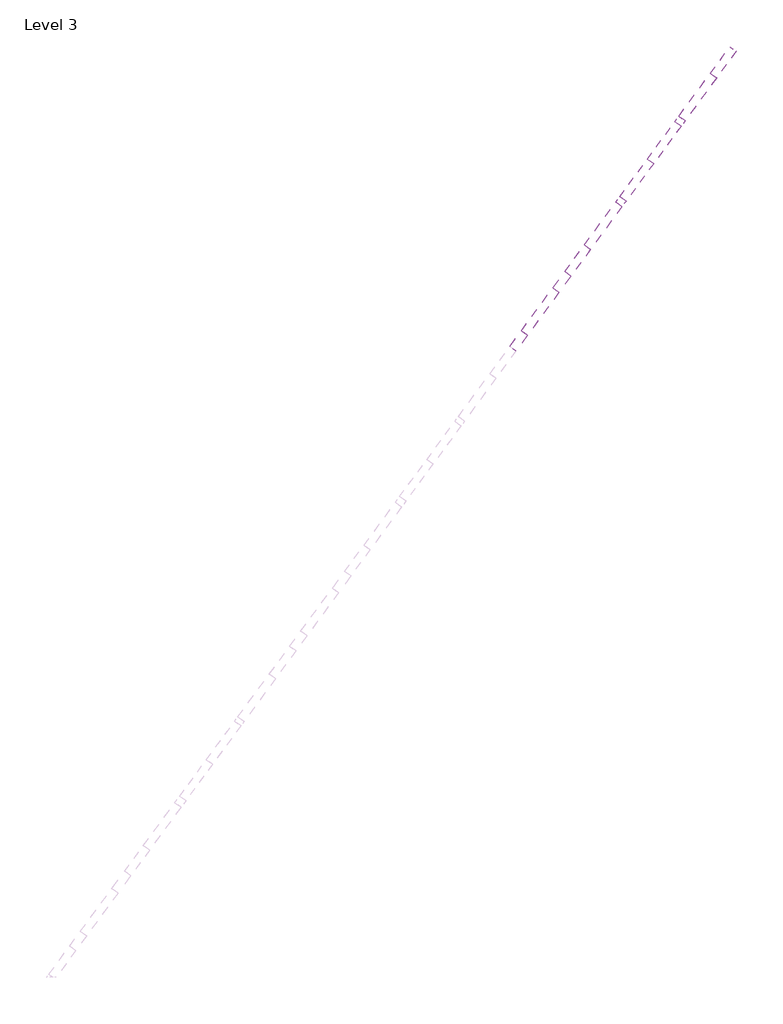
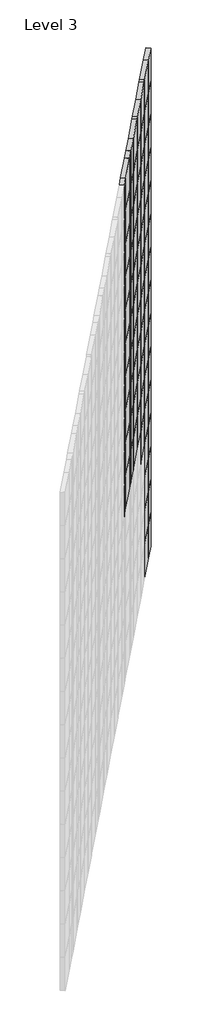
# One storey, part 9 of 9: 122 plates.
"""IFC4 building model written with IfcOpenShell, lengths in millimetres."""

import ifcopenshell
import ifcopenshell.guid

model = None  # the IFC model being written
_history = None  # IfcOwnerHistory: only IFC2X3 demands one
_inside = {}  # id of a spatial element -> (the spatial element, [elements in it])
_under = {}  # id of a project, library or spatial element -> (it, [spatial elements below it])
_declared = {}  # id of a project -> (the project, [libraries it declares])
_typed = {}  # id of a type object -> (the type object, [elements of that type])
_made_of = {}  # id of a material, layer set ... -> (it, [elements and type objects made of it])


def new_model(schema):
    """Start an empty IFC model of exactly this schema.

    Asked for "IFC4X3", IfcOpenShell would pick the latest addendum, in which some entities
    have other attributes; the version numbers below select the first issue.
    IFC2X3 requires an IfcOwnerHistory on every rooted entity: one is made here for all.
    """
    global model, _history
    if schema == "IFC4X3":
        model = ifcopenshell.file(schema_version=(4, 3, 0, 0))
    else:
        model = ifcopenshell.file(schema=schema)
    _inside.clear()
    _under.clear()
    _declared.clear()
    _typed.clear()
    _made_of.clear()
    _history = None
    if model.schema == "IFC2X3":
        org = make("IfcOrganization", Name="unknown")
        user = make(
            "IfcPersonAndOrganization",
            ThePerson=make("IfcPerson", FamilyName="unknown"),
            TheOrganization=org,
        )
        app = make(
            "IfcApplication",
            ApplicationDeveloper=org,
            Version="unknown",
            ApplicationFullName="unknown",
            ApplicationIdentifier="unknown",
        )
        _history = make(
            "IfcOwnerHistory",
            OwningUser=user,
            OwningApplication=app,
            ChangeAction="ADDED",
            CreationDate=0,
        )
    return model


def make(cls, **values):
    """One entity of the class cls with the attributes given. An attribute that is None is left unset."""
    return model.create_entity(
        cls, **{name: value for name, value in values.items() if value is not None}
    )


def rooted(cls, **values):
    """An entity with a GlobalId (a new one), such as an element, a storey or a relation."""
    return make(cls, GlobalId=ifcopenshell.guid.new(), OwnerHistory=_history, **values)


def si_unit(unit_type, name, prefix=None):
    """IfcSIUnit, for example si_unit("LENGTHUNIT", "METRE", prefix="MILLI")."""
    return make("IfcSIUnit", UnitType=unit_type, Prefix=prefix, Name=name)


def assignment(units):
    """IfcUnitAssignment: the units of a project."""
    return None if units is None else make("IfcUnitAssignment", Units=units)


def point(xyz):
    """IfcCartesianPoint."""
    return None if xyz is None else make("IfcCartesianPoint", Coordinates=xyz)


def direction(xyz):
    """IfcDirection."""
    return None if xyz is None else make("IfcDirection", DirectionRatios=xyz)


def frame(location, z_axis=None, x_axis=None):
    """IfcAxis2Placement3D, a coordinate frame: its origin and axes. An axis left out is left unset."""
    return make(
        "IfcAxis2Placement3D",
        Location=point(location),
        Axis=direction(z_axis),
        RefDirection=direction(x_axis),
    )


def origin():
    """The frame at (0, 0, 0) with its axes left unset."""
    return frame((0.0, 0.0, 0.0))


def origin_with_axes():
    """The frame at (0, 0, 0) with the z axis (0, 0, 1) and the x axis (1, 0, 0) written out."""
    return frame((0.0, 0.0, 0.0), z_axis=(0.0, 0.0, 1.0), x_axis=(1.0, 0.0, 0.0))


def place(relative_to, where):
    """IfcLocalPlacement: puts the frame where relative to a parent placement (None: the world)."""
    return make(
        "IfcLocalPlacement", PlacementRelTo=relative_to, RelativePlacement=where
    )


def context(
    kind, dimensions, precision=None, world=None, true_north=None, identifier=None
):
    """IfcGeometricRepresentationContext, for example the 3D "Model" context."""
    return make(
        "IfcGeometricRepresentationContext",
        ContextIdentifier=identifier,
        ContextType=kind,
        CoordinateSpaceDimension=dimensions,
        Precision=precision,
        WorldCoordinateSystem=world,
        TrueNorth=true_north,
    )


def project(units=None, contexts=None):
    """IfcProject with its units and contexts."""
    return rooted(
        "IfcProject",
        Name="project",
        RepresentationContexts=contexts,
        UnitsInContext=assignment(units),
    )


def spatial(cls, under=None, at=None, **own):
    """A site, building, storey or space (cls), placed at a placement, below another one or the project."""
    s = rooted(cls, ObjectPlacement=at, **own)
    if under is not None:
        _under.setdefault(under.id(), (under, []))[1].append(s)
    return s


def polyline(points):
    """IfcPolyline through the points."""
    return make("IfcPolyline", Points=[point(p) for p in points])


def outline(outer, holes=None, kind="AREA"):
    """IfcArbitraryClosedProfileDef: a profile drawn as a closed curve; with holes, ...WithVoids."""
    if holes is None:
        return make("IfcArbitraryClosedProfileDef", ProfileType=kind, OuterCurve=outer)
    return make(
        "IfcArbitraryProfileDefWithVoids",
        ProfileType=kind,
        OuterCurve=outer,
        InnerCurves=holes,
    )


def extrude(swept, where, along, depth):
    """IfcExtrudedAreaSolid: the profile swept, set in the frame where, extruded along a direction by depth."""
    return make(
        "IfcExtrudedAreaSolid",
        SweptArea=swept,
        Position=where,
        ExtrudedDirection=direction(along),
        Depth=depth,
    )


def shape(context_of_items, identifier, shape_type, items):
    """IfcShapeRepresentation: the items that make up one representation, for example the "Body"."""
    return make(
        "IfcShapeRepresentation",
        ContextOfItems=context_of_items,
        RepresentationIdentifier=identifier,
        RepresentationType=shape_type,
        Items=items,
    )


def source(mapping_origin, context_of_items, identifier, shape_type, items):
    """IfcRepresentationMap: a shape defined once, which mapped items show again and again."""
    return make(
        "IfcRepresentationMap",
        MappingOrigin=mapping_origin,
        MappedRepresentation=shape(context_of_items, identifier, shape_type, items),
    )


def transform(
    local_origin,
    x_axis=None,
    y_axis=None,
    z_axis=None,
    scale=None,
    scale2=None,
    scale3=None,
    uniform=True,
):
    """IfcCartesianTransformationOperator3D, or its non-uniform kind. x_axis, y_axis, z_axis: its Axis1, 2, 3."""
    if uniform:
        return make(
            "IfcCartesianTransformationOperator3D",
            Axis1=direction(x_axis),
            Axis2=direction(y_axis),
            LocalOrigin=point(local_origin),
            Scale=scale,
            Axis3=direction(z_axis),
        )
    return make(
        "IfcCartesianTransformationOperator3DnonUniform",
        Axis1=direction(x_axis),
        Axis2=direction(y_axis),
        LocalOrigin=point(local_origin),
        Scale=scale,
        Axis3=direction(z_axis),
        Scale2=scale2,
        Scale3=scale3,
    )


def mapped(mapping_source, mapping_target):
    """IfcMappedItem: shows the shape of a source again, moved by a transform."""
    return make(
        "IfcMappedItem", MappingSource=mapping_source, MappingTarget=mapping_target
    )


def made_of(thing, what):
    """Note that an element or type object is made of a material, layer set ...; save() writes the relation."""
    if what is not None:
        _made_of.setdefault(what.id(), (what, []))[1].append(thing)
    return thing


def element(
    cls,
    number,
    at=None,
    inside=None,
    cuts=None,
    type_object=None,
    material=None,
    context=None,
    identifier="Body",
    shape_type=None,
    held_by="IfcProductDefinitionShape",
    body=None,
    shapes=None,
    **own,
):
    """One element of the class cls, such as IfcWall. Its Tag is "e" and its number.

    at: its placement. inside: the storey or other place that contains it. cuts: it is an
    opening in that element (IfcRelVoidsElement). A single representation is given by context,
    identifier, shape_type and body (its items); several are given by shapes. held_by: the class
    of the entity that holds the representations. save() writes the other relations.
    """
    e = rooted(cls, Tag="e%d" % number, ObjectPlacement=at, **own)
    if body is not None:
        shapes = [shape(context, identifier, shape_type, body)]
    if shapes is not None:
        e.Representation = make(held_by, Representations=shapes)
    if inside is not None:
        _inside.setdefault(inside.id(), (inside, []))[1].append(e)
    if cuts is not None:
        rooted(
            "IfcRelVoidsElement", RelatingBuildingElement=cuts, RelatedOpeningElement=e
        )
    if type_object is not None:
        _typed.setdefault(type_object.id(), (type_object, []))[1].append(e)
    return made_of(e, material)


def aggregate(whole, parts):
    """IfcRelAggregates: a whole, such as a stair, and the parts it consists of."""
    return rooted("IfcRelAggregates", RelatingObject=whole, RelatedObjects=parts)


def save(model, path):
    """Write the relations noted so far, then the file.

    IfcRelAggregates (storeys below a building ...), IfcRelContainedInSpatialStructure (elements
    in a storey), IfcRelDefinesByType, IfcRelAssociatesMaterial and IfcRelDeclares: one each for
    every whole, place, type object, material and project.
    """
    for whole, parts in _under.values():
        aggregate(whole, parts)
    for where, things in _inside.values():
        rooted(
            "IfcRelContainedInSpatialStructure",
            RelatedElements=things,
            RelatingStructure=where,
        )
    for kind, things in _typed.values():
        rooted("IfcRelDefinesByType", RelatedObjects=things, RelatingType=kind)
    for what, things in _made_of.values():
        rooted("IfcRelAssociatesMaterial", RelatedObjects=things, RelatingMaterial=what)
    for by, libraries in _declared.values():
        rooted("IfcRelDeclares", RelatingContext=by, RelatedDefinitions=libraries)
    model.write(path)


def system_panel_glazed_6880485c(model_context):
    return source(origin(), model_context, "Body", "SweptSolid", [
        extrude(outline(polyline([(31.120151, 24.5), (-31.120151, 24.5), (-31.120151, 49.5), (31.120151, 49.5), (31.120151, 24.5)])), origin_with_axes(), (0.0, 0.0, 1.0), 200.0),
    ])


def system_panel_glazed_65218e73(model_context):
    return source(origin(), model_context, "Body", "SweptSolid", [
        extrude(outline(polyline([(52.6369119, 24.5), (-52.6369119, 24.5), (-52.6369119, 49.5), (52.6369119, 49.5), (52.6369119, 24.5)])), origin_with_axes(), (0.0, 0.0, 1.0), 200.0),
    ])


def system_panel_glazed_2ba9a9ff(model_context):
    return source(origin(), model_context, "Body", "SweptSolid", [
        extrude(outline(polyline([(74.1536727, 24.5), (-74.1536727, 24.5), (-74.1536727, 49.5), (74.1536727, 49.5), (74.1536727, 24.5)])), origin_with_axes(), (0.0, 0.0, 1.0), 200.0),
    ])


def system_panel_glazed_87147500(model_context):
    return source(origin(), model_context, "Body", "SweptSolid", [
        extrude(outline(polyline([(10.6704335, 24.5), (-10.6704335, 24.5), (-10.6704335, 49.5), (10.6704335, 49.5), (10.6704335, 24.5)])), origin_with_axes(), (0.0, 0.0, 1.0), 200.0),
    ])


def system_panel_glazed_1ea8d406(model_context):
    return source(origin(), model_context, "Body", "SweptSolid", [
        extrude(outline(polyline([(85.0, 24.5), (-85.0, 24.5), (-85.0, 49.5), (85.0, 49.5), (85.0, 24.5)])), origin_with_axes(), (0.0, 0.0, 1.0), 200.0),
    ])


def system_panel_glazed_d23853e5(model_context):
    return source(origin(), model_context, "Body", "SweptSolid", [
        extrude(outline(polyline([(32.3630881, 24.5), (-32.3630881, 24.5), (-32.3630881, 49.5), (32.3630881, 49.5), (32.3630881, 24.5)])), origin_with_axes(), (0.0, 0.0, 1.0), 200.0),
    ])


def system_panel_glazed_c2638314(model_context):
    return source(origin(), model_context, "Body", "SweptSolid", [
        extrude(outline(polyline([(10.8463273, 24.5), (-10.8463273, 24.5), (-10.8463273, 49.5), (10.8463273, 49.5), (10.8463273, 24.5)])), origin_with_axes(), (0.0, 0.0, 1.0), 200.0),
    ])


def system_panel_glazed_937a8ef3(model_context):
    return source(origin(), model_context, "Body", "SweptSolid", [
        extrude(outline(polyline([(74.3295665, 24.5), (-74.3295665, 24.5), (-74.3295665, 49.5), (74.3295665, 49.5), (74.3295665, 24.5)])), origin_with_axes(), (0.0, 0.0, 1.0), 200.0),
    ])


def system_panel_glazed_969c784e(model_context):
    return source(origin(), model_context, "Body", "SweptSolid", [
        extrude(outline(polyline([(52.8128058, 24.5), (-52.8128058, 24.5), (-52.8128058, 49.5), (52.8128058, 49.5), (52.8128058, 24.5)])), origin_with_axes(), (0.0, 0.0, 1.0), 200.0),
    ])


model = new_model("IFC4")

# Units and contexts
model_context = context("Model", 3, world=origin())
ifc_project = project(units=[si_unit("LENGTHUNIT", "METRE", prefix="MILLI")], contexts=[model_context])

# Site, building, storey
site = spatial("IfcSite", under=ifc_project)
building = spatial("IfcBuilding", under=site)
storey = spatial("IfcBuildingStorey", under=building, Name="Level 3", Elevation=22950.0)

# Plates
placement = place(None, origin())
system_panel_glazed_shape = system_panel_glazed_6880485c(model_context)
element("IfcPlate", 1, ObjectType="System Panel : Glazed", at=placement, inside=storey, context=model_context, shape_type="MappedRepresentation", body=[
    mapped(system_panel_glazed_shape, transform((-30980.4925467, 31282.997668, 36100.0), x_axis=(0.5920548138930122, 0.8058976965757569, 0.0), y_axis=(-0.8058976965757569, 0.5920548138930122, 0.0), z_axis=(0.0, 0.0, 1.0))),
])
element("IfcPlate", 2, ObjectType="System Panel : Glazed", at=placement, inside=storey, context=model_context, shape_type="MappedRepresentation", body=[
    mapped(system_panel_glazed_shape, transform((-30980.4925467, 31282.997668, 36300.0), x_axis=(0.5920548138930122, 0.8058976965757569, 0.0), y_axis=(-0.8058976965757569, 0.5920548138930122, 0.0), z_axis=(0.0, 0.0, 1.0))),
])
element("IfcPlate", 3, ObjectType="System Panel : Glazed", at=placement, inside=storey, context=model_context, shape_type="MappedRepresentation", body=[
    mapped(system_panel_glazed_shape, transform((-30980.4925467, 31282.997668, 36500.0), x_axis=(0.5920548138930122, 0.8058976965757569, 0.0), y_axis=(-0.8058976965757569, 0.5920548138930122, 0.0), z_axis=(0.0, 0.0, 1.0))),
])
element("IfcPlate", 4, ObjectType="System Panel : Glazed", at=placement, inside=storey, context=model_context, shape_type="MappedRepresentation", body=[
    mapped(system_panel_glazed_shape, transform((-30980.4925467, 31282.997668, 36700.0), x_axis=(0.5920548138930122, 0.8058976965757569, 0.0), y_axis=(-0.8058976965757569, 0.5920548138930122, 0.0), z_axis=(0.0, 0.0, 1.0))),
])
element("IfcPlate", 5, ObjectType="System Panel : Glazed", at=placement, inside=storey, context=model_context, shape_type="MappedRepresentation", body=[
    mapped(system_panel_glazed_shape, transform((-30980.4925467, 31282.997668, 36900.0), x_axis=(0.5920548138930122, 0.8058976965757569, 0.0), y_axis=(-0.8058976965757569, 0.5920548138930122, 0.0), z_axis=(0.0, 0.0, 1.0))),
])
element("IfcPlate", 6, ObjectType="System Panel : Glazed", at=placement, inside=storey, context=model_context, shape_type="MappedRepresentation", body=[
    mapped(system_panel_glazed_shape, transform((-30980.4925467, 31282.997668, 37100.0), x_axis=(0.5920548138930122, 0.8058976965757569, 0.0), y_axis=(-0.8058976965757569, 0.5920548138930122, 0.0), z_axis=(0.0, 0.0, 1.0))),
])
element("IfcPlate", 7, ObjectType="System Panel : Glazed", at=placement, inside=storey, context=model_context, shape_type="MappedRepresentation", body=[
    mapped(system_panel_glazed_shape, transform((-30980.4925467, 31282.997668, 37300.0), x_axis=(0.5920548138930122, 0.8058976965757569, 0.0), y_axis=(-0.8058976965757569, 0.5920548138930122, 0.0), z_axis=(0.0, 0.0, 1.0))),
])
element("IfcPlate", 8, ObjectType="System Panel : Glazed", at=placement, inside=storey, context=model_context, shape_type="MappedRepresentation", body=[
    mapped(system_panel_glazed_shape, transform((-30980.4925467, 31282.997668, 37500.0), x_axis=(0.5920548138930122, 0.8058976965757569, 0.0), y_axis=(-0.8058976965757569, 0.5920548138930122, 0.0), z_axis=(0.0, 0.0, 1.0))),
])
element("IfcPlate", 9, ObjectType="System Panel : Glazed", at=placement, inside=storey, context=model_context, shape_type="MappedRepresentation", body=[
    mapped(system_panel_glazed_shape, transform((-30980.4925467, 31282.997668, 37700.0), x_axis=(0.5920548138930122, 0.8058976965757569, 0.0), y_axis=(-0.8058976965757569, 0.5920548138930122, 0.0), z_axis=(0.0, 0.0, 1.0))),
])
element("IfcPlate", 10, ObjectType="System Panel : Glazed", at=placement, inside=storey, context=model_context, shape_type="MappedRepresentation", body=[
    mapped(system_panel_glazed_shape, transform((-30980.4925467, 31282.997668, 37900.0), x_axis=(0.5920548138930122, 0.8058976965757569, 0.0), y_axis=(-0.8058976965757569, 0.5920548138930122, 0.0), z_axis=(0.0, 0.0, 1.0))),
])
system_panel_glazed_2_shape = system_panel_glazed_65218e73(model_context)
element("IfcPlate", 11, ObjectType="System Panel : Glazed", at=placement, inside=storey, context=model_context, shape_type="MappedRepresentation", body=[
    mapped(system_panel_glazed_2_shape, transform((-30791.9330118, 31539.6625768, 36100.0), x_axis=(0.5920548138930122, 0.8058976965757569, 0.0), y_axis=(-0.8058976965757569, 0.5920548138930122, 0.0), z_axis=(0.0, 0.0, 1.0))),
])
element("IfcPlate", 12, ObjectType="System Panel : Glazed", at=placement, inside=storey, context=model_context, shape_type="MappedRepresentation", body=[
    mapped(system_panel_glazed_2_shape, transform((-30791.9330118, 31539.6625768, 36300.0), x_axis=(0.5920548138930122, 0.8058976965757569, 0.0), y_axis=(-0.8058976965757569, 0.5920548138930122, 0.0), z_axis=(0.0, 0.0, 1.0))),
])
element("IfcPlate", 13, ObjectType="System Panel : Glazed", at=placement, inside=storey, context=model_context, shape_type="MappedRepresentation", body=[
    mapped(system_panel_glazed_2_shape, transform((-30791.9330118, 31539.6625768, 36500.0), x_axis=(0.5920548138930122, 0.8058976965757569, 0.0), y_axis=(-0.8058976965757569, 0.5920548138930122, 0.0), z_axis=(0.0, 0.0, 1.0))),
])
element("IfcPlate", 14, ObjectType="System Panel : Glazed", at=placement, inside=storey, context=model_context, shape_type="MappedRepresentation", body=[
    mapped(system_panel_glazed_2_shape, transform((-30791.9330118, 31539.6625768, 36700.0), x_axis=(0.5920548138930122, 0.8058976965757569, 0.0), y_axis=(-0.8058976965757569, 0.5920548138930122, 0.0), z_axis=(0.0, 0.0, 1.0))),
])
element("IfcPlate", 15, ObjectType="System Panel : Glazed", at=placement, inside=storey, context=model_context, shape_type="MappedRepresentation", body=[
    mapped(system_panel_glazed_2_shape, transform((-30791.9330118, 31539.6625768, 36900.0), x_axis=(0.5920548138930122, 0.8058976965757569, 0.0), y_axis=(-0.8058976965757569, 0.5920548138930122, 0.0), z_axis=(0.0, 0.0, 1.0))),
])
element("IfcPlate", 16, ObjectType="System Panel : Glazed", at=placement, inside=storey, context=model_context, shape_type="MappedRepresentation", body=[
    mapped(system_panel_glazed_2_shape, transform((-30791.9330118, 31539.6625768, 37100.0), x_axis=(0.5920548138930122, 0.8058976965757569, 0.0), y_axis=(-0.8058976965757569, 0.5920548138930122, 0.0), z_axis=(0.0, 0.0, 1.0))),
])
element("IfcPlate", 17, ObjectType="System Panel : Glazed", at=placement, inside=storey, context=model_context, shape_type="MappedRepresentation", body=[
    mapped(system_panel_glazed_2_shape, transform((-30791.9330118, 31539.6625768, 37300.0), x_axis=(0.5920548138930122, 0.8058976965757569, 0.0), y_axis=(-0.8058976965757569, 0.5920548138930122, 0.0), z_axis=(0.0, 0.0, 1.0))),
])
element("IfcPlate", 18, ObjectType="System Panel : Glazed", at=placement, inside=storey, context=model_context, shape_type="MappedRepresentation", body=[
    mapped(system_panel_glazed_2_shape, transform((-30791.9330118, 31539.6625768, 37500.0), x_axis=(0.5920548138930122, 0.8058976965757569, 0.0), y_axis=(-0.8058976965757569, 0.5920548138930122, 0.0), z_axis=(0.0, 0.0, 1.0))),
])
element("IfcPlate", 19, ObjectType="System Panel : Glazed", at=placement, inside=storey, context=model_context, shape_type="MappedRepresentation", body=[
    mapped(system_panel_glazed_2_shape, transform((-30791.9330118, 31539.6625768, 37700.0), x_axis=(0.5920548138930122, 0.8058976965757569, 0.0), y_axis=(-0.8058976965757569, 0.5920548138930122, 0.0), z_axis=(0.0, 0.0, 1.0))),
])
element("IfcPlate", 20, ObjectType="System Panel : Glazed", at=placement, inside=storey, context=model_context, shape_type="MappedRepresentation", body=[
    mapped(system_panel_glazed_2_shape, transform((-30791.9330118, 31539.6625768, 37900.0), x_axis=(0.5920548138930122, 0.8058976965757569, 0.0), y_axis=(-0.8058976965757569, 0.5920548138930122, 0.0), z_axis=(0.0, 0.0, 1.0))),
])
system_panel_glazed_3_shape = system_panel_glazed_2ba9a9ff(model_context)
element("IfcPlate", 21, ObjectType="System Panel : Glazed", at=placement, inside=storey, context=model_context, shape_type="MappedRepresentation", body=[
    mapped(system_panel_glazed_3_shape, transform((-30603.373477, 31796.3274856, 36100.0), x_axis=(0.5920548138930122, 0.8058976965757569, 0.0), y_axis=(-0.8058976965757569, 0.5920548138930122, 0.0), z_axis=(0.0, 0.0, 1.0))),
])
element("IfcPlate", 22, ObjectType="System Panel : Glazed", at=placement, inside=storey, context=model_context, shape_type="MappedRepresentation", body=[
    mapped(system_panel_glazed_3_shape, transform((-30603.373477, 31796.3274856, 36300.0), x_axis=(0.5920548138930122, 0.8058976965757569, 0.0), y_axis=(-0.8058976965757569, 0.5920548138930122, 0.0), z_axis=(0.0, 0.0, 1.0))),
])
element("IfcPlate", 23, ObjectType="System Panel : Glazed", at=placement, inside=storey, context=model_context, shape_type="MappedRepresentation", body=[
    mapped(system_panel_glazed_3_shape, transform((-30603.373477, 31796.3274856, 36500.0), x_axis=(0.5920548138930122, 0.8058976965757569, 0.0), y_axis=(-0.8058976965757569, 0.5920548138930122, 0.0), z_axis=(0.0, 0.0, 1.0))),
])
element("IfcPlate", 24, ObjectType="System Panel : Glazed", at=placement, inside=storey, context=model_context, shape_type="MappedRepresentation", body=[
    mapped(system_panel_glazed_3_shape, transform((-30603.373477, 31796.3274856, 36700.0), x_axis=(0.5920548138930122, 0.8058976965757569, 0.0), y_axis=(-0.8058976965757569, 0.5920548138930122, 0.0), z_axis=(0.0, 0.0, 1.0))),
])
element("IfcPlate", 25, ObjectType="System Panel : Glazed", at=placement, inside=storey, context=model_context, shape_type="MappedRepresentation", body=[
    mapped(system_panel_glazed_3_shape, transform((-30603.373477, 31796.3274856, 36900.0), x_axis=(0.5920548138930122, 0.8058976965757569, 0.0), y_axis=(-0.8058976965757569, 0.5920548138930122, 0.0), z_axis=(0.0, 0.0, 1.0))),
])
element("IfcPlate", 26, ObjectType="System Panel : Glazed", at=placement, inside=storey, context=model_context, shape_type="MappedRepresentation", body=[
    mapped(system_panel_glazed_3_shape, transform((-30603.373477, 31796.3274856, 37100.0), x_axis=(0.5920548138930122, 0.8058976965757569, 0.0), y_axis=(-0.8058976965757569, 0.5920548138930122, 0.0), z_axis=(0.0, 0.0, 1.0))),
])
element("IfcPlate", 27, ObjectType="System Panel : Glazed", at=placement, inside=storey, context=model_context, shape_type="MappedRepresentation", body=[
    mapped(system_panel_glazed_3_shape, transform((-30603.373477, 31796.3274856, 37300.0), x_axis=(0.5920548138930122, 0.8058976965757569, 0.0), y_axis=(-0.8058976965757569, 0.5920548138930122, 0.0), z_axis=(0.0, 0.0, 1.0))),
])
element("IfcPlate", 28, ObjectType="System Panel : Glazed", at=placement, inside=storey, context=model_context, shape_type="MappedRepresentation", body=[
    mapped(system_panel_glazed_3_shape, transform((-30603.373477, 31796.3274856, 37500.0), x_axis=(0.5920548138930122, 0.8058976965757569, 0.0), y_axis=(-0.8058976965757569, 0.5920548138930122, 0.0), z_axis=(0.0, 0.0, 1.0))),
])
element("IfcPlate", 29, ObjectType="System Panel : Glazed", at=placement, inside=storey, context=model_context, shape_type="MappedRepresentation", body=[
    mapped(system_panel_glazed_3_shape, transform((-30603.373477, 31796.3274856, 37700.0), x_axis=(0.5920548138930122, 0.8058976965757569, 0.0), y_axis=(-0.8058976965757569, 0.5920548138930122, 0.0), z_axis=(0.0, 0.0, 1.0))),
])
element("IfcPlate", 30, ObjectType="System Panel : Glazed", at=placement, inside=storey, context=model_context, shape_type="MappedRepresentation", body=[
    mapped(system_panel_glazed_3_shape, transform((-30603.373477, 31796.3274856, 37900.0), x_axis=(0.5920548138930122, 0.8058976965757569, 0.0), y_axis=(-0.8058976965757569, 0.5920548138930122, 0.0), z_axis=(0.0, 0.0, 1.0))),
])
system_panel_glazed_4_shape = system_panel_glazed_87147500(model_context)
element("IfcPlate", 31, ObjectType="System Panel : Glazed", at=placement, inside=storey, context=model_context, shape_type="MappedRepresentation", body=[
    mapped(system_panel_glazed_4_shape, transform((-30465.1386012, 31984.4910903, 35900.0), x_axis=(0.5920548138930122, 0.8058976965757569, 0.0), y_axis=(-0.8058976965757569, 0.5920548138930122, 0.0), z_axis=(0.0, 0.0, 1.0))),
])
element("IfcPlate", 32, ObjectType="System Panel : Glazed", at=placement, inside=storey, context=model_context, shape_type="MappedRepresentation", body=[
    mapped(system_panel_glazed_4_shape, transform((-30465.1386012, 31984.4910903, 36100.0), x_axis=(0.5920548138930122, 0.8058976965757569, 0.0), y_axis=(-0.8058976965757569, 0.5920548138930122, 0.0), z_axis=(0.0, 0.0, 1.0))),
])
element("IfcPlate", 33, ObjectType="System Panel : Glazed", at=placement, inside=storey, context=model_context, shape_type="MappedRepresentation", body=[
    mapped(system_panel_glazed_4_shape, transform((-30465.1386012, 31984.4910903, 36300.0), x_axis=(0.5920548138930122, 0.8058976965757569, 0.0), y_axis=(-0.8058976965757569, 0.5920548138930122, 0.0), z_axis=(0.0, 0.0, 1.0))),
])
element("IfcPlate", 34, ObjectType="System Panel : Glazed", at=placement, inside=storey, context=model_context, shape_type="MappedRepresentation", body=[
    mapped(system_panel_glazed_4_shape, transform((-30465.1386012, 31984.4910903, 36500.0), x_axis=(0.5920548138930122, 0.8058976965757569, 0.0), y_axis=(-0.8058976965757569, 0.5920548138930122, 0.0), z_axis=(0.0, 0.0, 1.0))),
])
element("IfcPlate", 35, ObjectType="System Panel : Glazed", at=placement, inside=storey, context=model_context, shape_type="MappedRepresentation", body=[
    mapped(system_panel_glazed_4_shape, transform((-30465.1386012, 31984.4910903, 36700.0), x_axis=(0.5920548138930122, 0.8058976965757569, 0.0), y_axis=(-0.8058976965757569, 0.5920548138930122, 0.0), z_axis=(0.0, 0.0, 1.0))),
])
element("IfcPlate", 36, ObjectType="System Panel : Glazed", at=placement, inside=storey, context=model_context, shape_type="MappedRepresentation", body=[
    mapped(system_panel_glazed_4_shape, transform((-30465.1386012, 31984.4910903, 36900.0), x_axis=(0.5920548138930122, 0.8058976965757569, 0.0), y_axis=(-0.8058976965757569, 0.5920548138930122, 0.0), z_axis=(0.0, 0.0, 1.0))),
])
element("IfcPlate", 37, ObjectType="System Panel : Glazed", at=placement, inside=storey, context=model_context, shape_type="MappedRepresentation", body=[
    mapped(system_panel_glazed_4_shape, transform((-30465.1386012, 31984.4910903, 37100.0), x_axis=(0.5920548138930122, 0.8058976965757569, 0.0), y_axis=(-0.8058976965757569, 0.5920548138930122, 0.0), z_axis=(0.0, 0.0, 1.0))),
])
element("IfcPlate", 38, ObjectType="System Panel : Glazed", at=placement, inside=storey, context=model_context, shape_type="MappedRepresentation", body=[
    mapped(system_panel_glazed_4_shape, transform((-30465.1386012, 31984.4910903, 37300.0), x_axis=(0.5920548138930122, 0.8058976965757569, 0.0), y_axis=(-0.8058976965757569, 0.5920548138930122, 0.0), z_axis=(0.0, 0.0, 1.0))),
])
element("IfcPlate", 39, ObjectType="System Panel : Glazed", at=placement, inside=storey, context=model_context, shape_type="MappedRepresentation", body=[
    mapped(system_panel_glazed_4_shape, transform((-30465.1386012, 31984.4910903, 37500.0), x_axis=(0.5920548138930122, 0.8058976965757569, 0.0), y_axis=(-0.8058976965757569, 0.5920548138930122, 0.0), z_axis=(0.0, 0.0, 1.0))),
])
element("IfcPlate", 40, ObjectType="System Panel : Glazed", at=placement, inside=storey, context=model_context, shape_type="MappedRepresentation", body=[
    mapped(system_panel_glazed_4_shape, transform((-30465.1386012, 31984.4910903, 37700.0), x_axis=(0.5920548138930122, 0.8058976965757569, 0.0), y_axis=(-0.8058976965757569, 0.5920548138930122, 0.0), z_axis=(0.0, 0.0, 1.0))),
])
element("IfcPlate", 41, ObjectType="System Panel : Glazed", at=placement, inside=storey, context=model_context, shape_type="MappedRepresentation", body=[
    mapped(system_panel_glazed_4_shape, transform((-30465.1386012, 31984.4910903, 37900.0), x_axis=(0.5920548138930122, 0.8058976965757569, 0.0), y_axis=(-0.8058976965757569, 0.5920548138930122, 0.0), z_axis=(0.0, 0.0, 1.0))),
])
system_panel_glazed_5_shape = system_panel_glazed_1ea8d406(model_context)
element("IfcPlate", 42, ObjectType="System Panel : Glazed", at=placement, inside=storey, context=model_context, shape_type="MappedRepresentation", body=[
    mapped(system_panel_glazed_5_shape, transform((-30408.4964605, 32061.5916723, 35100.0), x_axis=(0.5920548138930122, 0.8058976965757569, 0.0), y_axis=(-0.8058976965757569, 0.5920548138930122, 0.0), z_axis=(0.0, 0.0, 1.0))),
])
element("IfcPlate", 43, ObjectType="System Panel : Glazed", at=placement, inside=storey, context=model_context, shape_type="MappedRepresentation", body=[
    mapped(system_panel_glazed_5_shape, transform((-30408.4964605, 32061.5916723, 35300.0), x_axis=(0.5920548138930122, 0.8058976965757569, 0.0), y_axis=(-0.8058976965757569, 0.5920548138930122, 0.0), z_axis=(0.0, 0.0, 1.0))),
])
element("IfcPlate", 44, ObjectType="System Panel : Glazed", at=placement, inside=storey, context=model_context, shape_type="MappedRepresentation", body=[
    mapped(system_panel_glazed_5_shape, transform((-30408.4964605, 32061.5916723, 35500.0), x_axis=(0.5920548138930122, 0.8058976965757569, 0.0), y_axis=(-0.8058976965757569, 0.5920548138930122, 0.0), z_axis=(0.0, 0.0, 1.0))),
])
element("IfcPlate", 45, ObjectType="System Panel : Glazed", at=placement, inside=storey, context=model_context, shape_type="MappedRepresentation", body=[
    mapped(system_panel_glazed_5_shape, transform((-30408.4964605, 32061.5916723, 35700.0), x_axis=(0.5920548138930122, 0.8058976965757569, 0.0), y_axis=(-0.8058976965757569, 0.5920548138930122, 0.0), z_axis=(0.0, 0.0, 1.0))),
])
element("IfcPlate", 46, ObjectType="System Panel : Glazed", at=placement, inside=storey, context=model_context, shape_type="MappedRepresentation", body=[
    mapped(system_panel_glazed_5_shape, transform((-30408.4964605, 32061.5916723, 35900.0), x_axis=(0.5920548138930122, 0.8058976965757569, 0.0), y_axis=(-0.8058976965757569, 0.5920548138930122, 0.0), z_axis=(0.0, 0.0, 1.0))),
])
element("IfcPlate", 47, ObjectType="System Panel : Glazed", at=placement, inside=storey, context=model_context, shape_type="MappedRepresentation", body=[
    mapped(system_panel_glazed_5_shape, transform((-30911.7430523, 31376.5786302, 36100.0), x_axis=(0.5920548138930122, 0.8058976965757569, 0.0), y_axis=(-0.8058976965757569, 0.5920548138930122, 0.0), z_axis=(0.0, 0.0, 1.0))),
])
element("IfcPlate", 48, ObjectType="System Panel : Glazed", at=placement, inside=storey, context=model_context, shape_type="MappedRepresentation", body=[
    mapped(system_panel_glazed_5_shape, transform((-30710.4444156, 31650.583847, 36100.0), x_axis=(0.5920548138930122, 0.8058976965757569, 0.0), y_axis=(-0.8058976965757569, 0.5920548138930122, 0.0), z_axis=(0.0, 0.0, 1.0))),
])
element("IfcPlate", 49, ObjectType="System Panel : Glazed", at=placement, inside=storey, context=model_context, shape_type="MappedRepresentation", body=[
    mapped(system_panel_glazed_5_shape, transform((-30408.4964605, 32061.5916723, 36100.0), x_axis=(0.5920548138930122, 0.8058976965757569, 0.0), y_axis=(-0.8058976965757569, 0.5920548138930122, 0.0), z_axis=(0.0, 0.0, 1.0))),
])
element("IfcPlate", 50, ObjectType="System Panel : Glazed", at=placement, inside=storey, context=model_context, shape_type="MappedRepresentation", body=[
    mapped(system_panel_glazed_5_shape, transform((-30911.7430523, 31376.5786302, 36300.0), x_axis=(0.5920548138930122, 0.8058976965757569, 0.0), y_axis=(-0.8058976965757569, 0.5920548138930122, 0.0), z_axis=(0.0, 0.0, 1.0))),
])
element("IfcPlate", 51, ObjectType="System Panel : Glazed", at=placement, inside=storey, context=model_context, shape_type="MappedRepresentation", body=[
    mapped(system_panel_glazed_5_shape, transform((-30710.4444156, 31650.583847, 36300.0), x_axis=(0.5920548138930122, 0.8058976965757569, 0.0), y_axis=(-0.8058976965757569, 0.5920548138930122, 0.0), z_axis=(0.0, 0.0, 1.0))),
])
element("IfcPlate", 52, ObjectType="System Panel : Glazed", at=placement, inside=storey, context=model_context, shape_type="MappedRepresentation", body=[
    mapped(system_panel_glazed_5_shape, transform((-30408.4964605, 32061.5916723, 36300.0), x_axis=(0.5920548138930122, 0.8058976965757569, 0.0), y_axis=(-0.8058976965757569, 0.5920548138930122, 0.0), z_axis=(0.0, 0.0, 1.0))),
])
element("IfcPlate", 53, ObjectType="System Panel : Glazed", at=placement, inside=storey, context=model_context, shape_type="MappedRepresentation", body=[
    mapped(system_panel_glazed_5_shape, transform((-30911.7430523, 31376.5786302, 36500.0), x_axis=(0.5920548138930122, 0.8058976965757569, 0.0), y_axis=(-0.8058976965757569, 0.5920548138930122, 0.0), z_axis=(0.0, 0.0, 1.0))),
])
element("IfcPlate", 54, ObjectType="System Panel : Glazed", at=placement, inside=storey, context=model_context, shape_type="MappedRepresentation", body=[
    mapped(system_panel_glazed_5_shape, transform((-30710.4444156, 31650.583847, 36500.0), x_axis=(0.5920548138930122, 0.8058976965757569, 0.0), y_axis=(-0.8058976965757569, 0.5920548138930122, 0.0), z_axis=(0.0, 0.0, 1.0))),
])
element("IfcPlate", 55, ObjectType="System Panel : Glazed", at=placement, inside=storey, context=model_context, shape_type="MappedRepresentation", body=[
    mapped(system_panel_glazed_5_shape, transform((-30408.4964605, 32061.5916723, 36500.0), x_axis=(0.5920548138930122, 0.8058976965757569, 0.0), y_axis=(-0.8058976965757569, 0.5920548138930122, 0.0), z_axis=(0.0, 0.0, 1.0))),
])
element("IfcPlate", 56, ObjectType="System Panel : Glazed", at=placement, inside=storey, context=model_context, shape_type="MappedRepresentation", body=[
    mapped(system_panel_glazed_5_shape, transform((-30911.7430523, 31376.5786302, 36700.0), x_axis=(0.5920548138930122, 0.8058976965757569, 0.0), y_axis=(-0.8058976965757569, 0.5920548138930122, 0.0), z_axis=(0.0, 0.0, 1.0))),
])
element("IfcPlate", 57, ObjectType="System Panel : Glazed", at=placement, inside=storey, context=model_context, shape_type="MappedRepresentation", body=[
    mapped(system_panel_glazed_5_shape, transform((-30710.4444156, 31650.583847, 36700.0), x_axis=(0.5920548138930122, 0.8058976965757569, 0.0), y_axis=(-0.8058976965757569, 0.5920548138930122, 0.0), z_axis=(0.0, 0.0, 1.0))),
])
element("IfcPlate", 58, ObjectType="System Panel : Glazed", at=placement, inside=storey, context=model_context, shape_type="MappedRepresentation", body=[
    mapped(system_panel_glazed_5_shape, transform((-30408.4964605, 32061.5916723, 36700.0), x_axis=(0.5920548138930122, 0.8058976965757569, 0.0), y_axis=(-0.8058976965757569, 0.5920548138930122, 0.0), z_axis=(0.0, 0.0, 1.0))),
])
element("IfcPlate", 59, ObjectType="System Panel : Glazed", at=placement, inside=storey, context=model_context, shape_type="MappedRepresentation", body=[
    mapped(system_panel_glazed_5_shape, transform((-30911.7430523, 31376.5786302, 36900.0), x_axis=(0.5920548138930122, 0.8058976965757569, 0.0), y_axis=(-0.8058976965757569, 0.5920548138930122, 0.0), z_axis=(0.0, 0.0, 1.0))),
])
element("IfcPlate", 60, ObjectType="System Panel : Glazed", at=placement, inside=storey, context=model_context, shape_type="MappedRepresentation", body=[
    mapped(system_panel_glazed_5_shape, transform((-30710.4444156, 31650.583847, 36900.0), x_axis=(0.5920548138930122, 0.8058976965757569, 0.0), y_axis=(-0.8058976965757569, 0.5920548138930122, 0.0), z_axis=(0.0, 0.0, 1.0))),
])
element("IfcPlate", 61, ObjectType="System Panel : Glazed", at=placement, inside=storey, context=model_context, shape_type="MappedRepresentation", body=[
    mapped(system_panel_glazed_5_shape, transform((-30408.4964605, 32061.5916723, 36900.0), x_axis=(0.5920548138930122, 0.8058976965757569, 0.0), y_axis=(-0.8058976965757569, 0.5920548138930122, 0.0), z_axis=(0.0, 0.0, 1.0))),
])
element("IfcPlate", 62, ObjectType="System Panel : Glazed", at=placement, inside=storey, context=model_context, shape_type="MappedRepresentation", body=[
    mapped(system_panel_glazed_5_shape, transform((-30911.7430523, 31376.5786302, 37100.0), x_axis=(0.5920548138930122, 0.8058976965757569, 0.0), y_axis=(-0.8058976965757569, 0.5920548138930122, 0.0), z_axis=(0.0, 0.0, 1.0))),
])
element("IfcPlate", 63, ObjectType="System Panel : Glazed", at=placement, inside=storey, context=model_context, shape_type="MappedRepresentation", body=[
    mapped(system_panel_glazed_5_shape, transform((-30710.4444156, 31650.583847, 37100.0), x_axis=(0.5920548138930122, 0.8058976965757569, 0.0), y_axis=(-0.8058976965757569, 0.5920548138930122, 0.0), z_axis=(0.0, 0.0, 1.0))),
])
element("IfcPlate", 64, ObjectType="System Panel : Glazed", at=placement, inside=storey, context=model_context, shape_type="MappedRepresentation", body=[
    mapped(system_panel_glazed_5_shape, transform((-30408.4964605, 32061.5916723, 37100.0), x_axis=(0.5920548138930122, 0.8058976965757569, 0.0), y_axis=(-0.8058976965757569, 0.5920548138930122, 0.0), z_axis=(0.0, 0.0, 1.0))),
])
element("IfcPlate", 65, ObjectType="System Panel : Glazed", at=placement, inside=storey, context=model_context, shape_type="MappedRepresentation", body=[
    mapped(system_panel_glazed_5_shape, transform((-30911.7430523, 31376.5786302, 37300.0), x_axis=(0.5920548138930122, 0.8058976965757569, 0.0), y_axis=(-0.8058976965757569, 0.5920548138930122, 0.0), z_axis=(0.0, 0.0, 1.0))),
])
element("IfcPlate", 66, ObjectType="System Panel : Glazed", at=placement, inside=storey, context=model_context, shape_type="MappedRepresentation", body=[
    mapped(system_panel_glazed_5_shape, transform((-30710.4444156, 31650.583847, 37300.0), x_axis=(0.5920548138930122, 0.8058976965757569, 0.0), y_axis=(-0.8058976965757569, 0.5920548138930122, 0.0), z_axis=(0.0, 0.0, 1.0))),
])
element("IfcPlate", 67, ObjectType="System Panel : Glazed", at=placement, inside=storey, context=model_context, shape_type="MappedRepresentation", body=[
    mapped(system_panel_glazed_5_shape, transform((-30408.4964605, 32061.5916723, 37300.0), x_axis=(0.5920548138930122, 0.8058976965757569, 0.0), y_axis=(-0.8058976965757569, 0.5920548138930122, 0.0), z_axis=(0.0, 0.0, 1.0))),
])
element("IfcPlate", 68, ObjectType="System Panel : Glazed", at=placement, inside=storey, context=model_context, shape_type="MappedRepresentation", body=[
    mapped(system_panel_glazed_5_shape, transform((-30911.7430523, 31376.5786302, 37500.0), x_axis=(0.5920548138930122, 0.8058976965757569, 0.0), y_axis=(-0.8058976965757569, 0.5920548138930122, 0.0), z_axis=(0.0, 0.0, 1.0))),
])
element("IfcPlate", 69, ObjectType="System Panel : Glazed", at=placement, inside=storey, context=model_context, shape_type="MappedRepresentation", body=[
    mapped(system_panel_glazed_5_shape, transform((-30710.4444156, 31650.583847, 37500.0), x_axis=(0.5920548138930122, 0.8058976965757569, 0.0), y_axis=(-0.8058976965757569, 0.5920548138930122, 0.0), z_axis=(0.0, 0.0, 1.0))),
])
element("IfcPlate", 70, ObjectType="System Panel : Glazed", at=placement, inside=storey, context=model_context, shape_type="MappedRepresentation", body=[
    mapped(system_panel_glazed_5_shape, transform((-30408.4964605, 32061.5916723, 37500.0), x_axis=(0.5920548138930122, 0.8058976965757569, 0.0), y_axis=(-0.8058976965757569, 0.5920548138930122, 0.0), z_axis=(0.0, 0.0, 1.0))),
])
element("IfcPlate", 71, ObjectType="System Panel : Glazed", at=placement, inside=storey, context=model_context, shape_type="MappedRepresentation", body=[
    mapped(system_panel_glazed_5_shape, transform((-30911.7430523, 31376.5786302, 37700.0), x_axis=(0.5920548138930122, 0.8058976965757569, 0.0), y_axis=(-0.8058976965757569, 0.5920548138930122, 0.0), z_axis=(0.0, 0.0, 1.0))),
])
element("IfcPlate", 72, ObjectType="System Panel : Glazed", at=placement, inside=storey, context=model_context, shape_type="MappedRepresentation", body=[
    mapped(system_panel_glazed_5_shape, transform((-30710.4444156, 31650.583847, 37700.0), x_axis=(0.5920548138930122, 0.8058976965757569, 0.0), y_axis=(-0.8058976965757569, 0.5920548138930122, 0.0), z_axis=(0.0, 0.0, 1.0))),
])
element("IfcPlate", 73, ObjectType="System Panel : Glazed", at=placement, inside=storey, context=model_context, shape_type="MappedRepresentation", body=[
    mapped(system_panel_glazed_5_shape, transform((-30408.4964605, 32061.5916723, 37700.0), x_axis=(0.5920548138930122, 0.8058976965757569, 0.0), y_axis=(-0.8058976965757569, 0.5920548138930122, 0.0), z_axis=(0.0, 0.0, 1.0))),
])
element("IfcPlate", 74, ObjectType="System Panel : Glazed", at=placement, inside=storey, context=model_context, shape_type="MappedRepresentation", body=[
    mapped(system_panel_glazed_5_shape, transform((-30911.7430523, 31376.5786302, 37900.0), x_axis=(0.5920548138930122, 0.8058976965757569, 0.0), y_axis=(-0.8058976965757569, 0.5920548138930122, 0.0), z_axis=(0.0, 0.0, 1.0))),
])
element("IfcPlate", 75, ObjectType="System Panel : Glazed", at=placement, inside=storey, context=model_context, shape_type="MappedRepresentation", body=[
    mapped(system_panel_glazed_5_shape, transform((-30710.4444156, 31650.583847, 37900.0), x_axis=(0.5920548138930122, 0.8058976965757569, 0.0), y_axis=(-0.8058976965757569, 0.5920548138930122, 0.0), z_axis=(0.0, 0.0, 1.0))),
])
element("IfcPlate", 76, ObjectType="System Panel : Glazed", at=placement, inside=storey, context=model_context, shape_type="MappedRepresentation", body=[
    mapped(system_panel_glazed_5_shape, transform((-30408.4964605, 32061.5916723, 37900.0), x_axis=(0.5920548138930122, 0.8058976965757569, 0.0), y_axis=(-0.8058976965757569, 0.5920548138930122, 0.0), z_axis=(0.0, 0.0, 1.0))),
])
system_panel_glazed_6_shape = system_panel_glazed_d23853e5(model_context)
element("IfcPlate", 77, ObjectType="System Panel : Glazed", at=placement, inside=storey, context=model_context, shape_type="MappedRepresentation", body=[
    mapped(system_panel_glazed_6_shape, transform((-30842.257671, 31471.1612726, 36100.0), x_axis=(0.5920548138930122, 0.8058976965757569, 0.0), y_axis=(-0.8058976965757569, 0.5920548138930122, 0.0), z_axis=(0.0, 0.0, 1.0))),
])
element("IfcPlate", 78, ObjectType="System Panel : Glazed", at=placement, inside=storey, context=model_context, shape_type="MappedRepresentation", body=[
    mapped(system_panel_glazed_6_shape, transform((-30842.257671, 31471.1612726, 36300.0), x_axis=(0.5920548138930122, 0.8058976965757569, 0.0), y_axis=(-0.8058976965757569, 0.5920548138930122, 0.0), z_axis=(0.0, 0.0, 1.0))),
])
element("IfcPlate", 79, ObjectType="System Panel : Glazed", at=placement, inside=storey, context=model_context, shape_type="MappedRepresentation", body=[
    mapped(system_panel_glazed_6_shape, transform((-30842.257671, 31471.1612726, 36500.0), x_axis=(0.5920548138930122, 0.8058976965757569, 0.0), y_axis=(-0.8058976965757569, 0.5920548138930122, 0.0), z_axis=(0.0, 0.0, 1.0))),
])
element("IfcPlate", 80, ObjectType="System Panel : Glazed", at=placement, inside=storey, context=model_context, shape_type="MappedRepresentation", body=[
    mapped(system_panel_glazed_6_shape, transform((-30842.257671, 31471.1612726, 36700.0), x_axis=(0.5920548138930122, 0.8058976965757569, 0.0), y_axis=(-0.8058976965757569, 0.5920548138930122, 0.0), z_axis=(0.0, 0.0, 1.0))),
])
element("IfcPlate", 81, ObjectType="System Panel : Glazed", at=placement, inside=storey, context=model_context, shape_type="MappedRepresentation", body=[
    mapped(system_panel_glazed_6_shape, transform((-30842.257671, 31471.1612726, 36900.0), x_axis=(0.5920548138930122, 0.8058976965757569, 0.0), y_axis=(-0.8058976965757569, 0.5920548138930122, 0.0), z_axis=(0.0, 0.0, 1.0))),
])
element("IfcPlate", 82, ObjectType="System Panel : Glazed", at=placement, inside=storey, context=model_context, shape_type="MappedRepresentation", body=[
    mapped(system_panel_glazed_6_shape, transform((-30842.257671, 31471.1612726, 37100.0), x_axis=(0.5920548138930122, 0.8058976965757569, 0.0), y_axis=(-0.8058976965757569, 0.5920548138930122, 0.0), z_axis=(0.0, 0.0, 1.0))),
])
element("IfcPlate", 83, ObjectType="System Panel : Glazed", at=placement, inside=storey, context=model_context, shape_type="MappedRepresentation", body=[
    mapped(system_panel_glazed_6_shape, transform((-30842.257671, 31471.1612726, 37300.0), x_axis=(0.5920548138930122, 0.8058976965757569, 0.0), y_axis=(-0.8058976965757569, 0.5920548138930122, 0.0), z_axis=(0.0, 0.0, 1.0))),
])
element("IfcPlate", 84, ObjectType="System Panel : Glazed", at=placement, inside=storey, context=model_context, shape_type="MappedRepresentation", body=[
    mapped(system_panel_glazed_6_shape, transform((-30842.257671, 31471.1612726, 37500.0), x_axis=(0.5920548138930122, 0.8058976965757569, 0.0), y_axis=(-0.8058976965757569, 0.5920548138930122, 0.0), z_axis=(0.0, 0.0, 1.0))),
])
element("IfcPlate", 85, ObjectType="System Panel : Glazed", at=placement, inside=storey, context=model_context, shape_type="MappedRepresentation", body=[
    mapped(system_panel_glazed_6_shape, transform((-30842.257671, 31471.1612726, 37700.0), x_axis=(0.5920548138930122, 0.8058976965757569, 0.0), y_axis=(-0.8058976965757569, 0.5920548138930122, 0.0), z_axis=(0.0, 0.0, 1.0))),
])
element("IfcPlate", 86, ObjectType="System Panel : Glazed", at=placement, inside=storey, context=model_context, shape_type="MappedRepresentation", body=[
    mapped(system_panel_glazed_6_shape, transform((-30842.257671, 31471.1612726, 37900.0), x_axis=(0.5920548138930122, 0.8058976965757569, 0.0), y_axis=(-0.8058976965757569, 0.5920548138930122, 0.0), z_axis=(0.0, 0.0, 1.0))),
])
system_panel_glazed_7_shape = system_panel_glazed_c2638314(model_context)
element("IfcPlate", 87, ObjectType="System Panel : Glazed", at=placement, inside=storey, context=model_context, shape_type="MappedRepresentation", body=[
    mapped(system_panel_glazed_7_shape, transform((-30653.6981361, 31727.8261814, 36100.0), x_axis=(0.5920548138930122, 0.8058976965757569, 0.0), y_axis=(-0.8058976965757569, 0.5920548138930122, 0.0), z_axis=(0.0, 0.0, 1.0))),
])
element("IfcPlate", 88, ObjectType="System Panel : Glazed", at=placement, inside=storey, context=model_context, shape_type="MappedRepresentation", body=[
    mapped(system_panel_glazed_7_shape, transform((-30653.6981361, 31727.8261814, 36300.0), x_axis=(0.5920548138930122, 0.8058976965757569, 0.0), y_axis=(-0.8058976965757569, 0.5920548138930122, 0.0), z_axis=(0.0, 0.0, 1.0))),
])
element("IfcPlate", 89, ObjectType="System Panel : Glazed", at=placement, inside=storey, context=model_context, shape_type="MappedRepresentation", body=[
    mapped(system_panel_glazed_7_shape, transform((-30653.6981361, 31727.8261814, 36500.0), x_axis=(0.5920548138930122, 0.8058976965757569, 0.0), y_axis=(-0.8058976965757569, 0.5920548138930122, 0.0), z_axis=(0.0, 0.0, 1.0))),
])
element("IfcPlate", 90, ObjectType="System Panel : Glazed", at=placement, inside=storey, context=model_context, shape_type="MappedRepresentation", body=[
    mapped(system_panel_glazed_7_shape, transform((-30653.6981361, 31727.8261814, 36700.0), x_axis=(0.5920548138930122, 0.8058976965757569, 0.0), y_axis=(-0.8058976965757569, 0.5920548138930122, 0.0), z_axis=(0.0, 0.0, 1.0))),
])
element("IfcPlate", 91, ObjectType="System Panel : Glazed", at=placement, inside=storey, context=model_context, shape_type="MappedRepresentation", body=[
    mapped(system_panel_glazed_7_shape, transform((-30653.6981361, 31727.8261814, 36900.0), x_axis=(0.5920548138930122, 0.8058976965757569, 0.0), y_axis=(-0.8058976965757569, 0.5920548138930122, 0.0), z_axis=(0.0, 0.0, 1.0))),
])
element("IfcPlate", 92, ObjectType="System Panel : Glazed", at=placement, inside=storey, context=model_context, shape_type="MappedRepresentation", body=[
    mapped(system_panel_glazed_7_shape, transform((-30653.6981361, 31727.8261814, 37100.0), x_axis=(0.5920548138930122, 0.8058976965757569, 0.0), y_axis=(-0.8058976965757569, 0.5920548138930122, 0.0), z_axis=(0.0, 0.0, 1.0))),
])
element("IfcPlate", 93, ObjectType="System Panel : Glazed", at=placement, inside=storey, context=model_context, shape_type="MappedRepresentation", body=[
    mapped(system_panel_glazed_7_shape, transform((-30653.6981361, 31727.8261814, 37300.0), x_axis=(0.5920548138930122, 0.8058976965757569, 0.0), y_axis=(-0.8058976965757569, 0.5920548138930122, 0.0), z_axis=(0.0, 0.0, 1.0))),
])
element("IfcPlate", 94, ObjectType="System Panel : Glazed", at=placement, inside=storey, context=model_context, shape_type="MappedRepresentation", body=[
    mapped(system_panel_glazed_7_shape, transform((-30653.6981361, 31727.8261814, 37500.0), x_axis=(0.5920548138930122, 0.8058976965757569, 0.0), y_axis=(-0.8058976965757569, 0.5920548138930122, 0.0), z_axis=(0.0, 0.0, 1.0))),
])
element("IfcPlate", 95, ObjectType="System Panel : Glazed", at=placement, inside=storey, context=model_context, shape_type="MappedRepresentation", body=[
    mapped(system_panel_glazed_7_shape, transform((-30653.6981361, 31727.8261814, 37700.0), x_axis=(0.5920548138930122, 0.8058976965757569, 0.0), y_axis=(-0.8058976965757569, 0.5920548138930122, 0.0), z_axis=(0.0, 0.0, 1.0))),
])
element("IfcPlate", 96, ObjectType="System Panel : Glazed", at=placement, inside=storey, context=model_context, shape_type="MappedRepresentation", body=[
    mapped(system_panel_glazed_7_shape, transform((-30653.6981361, 31727.8261814, 37900.0), x_axis=(0.5920548138930122, 0.8058976965757569, 0.0), y_axis=(-0.8058976965757569, 0.5920548138930122, 0.0), z_axis=(0.0, 0.0, 1.0))),
])
system_panel_glazed_8_shape = system_panel_glazed_937a8ef3(model_context)
element("IfcPlate", 97, ObjectType="System Panel : Glazed", at=placement, inside=storey, context=model_context, shape_type="MappedRepresentation", body=[
    mapped(system_panel_glazed_8_shape, transform((-30515.4632604, 31915.989786, 35900.0), x_axis=(0.5920548138930122, 0.8058976965757569, 0.0), y_axis=(-0.8058976965757569, 0.5920548138930122, 0.0), z_axis=(0.0, 0.0, 1.0))),
])
element("IfcPlate", 98, ObjectType="System Panel : Glazed", at=placement, inside=storey, context=model_context, shape_type="MappedRepresentation", body=[
    mapped(system_panel_glazed_8_shape, transform((-30515.4632604, 31915.989786, 36100.0), x_axis=(0.5920548138930122, 0.8058976965757569, 0.0), y_axis=(-0.8058976965757569, 0.5920548138930122, 0.0), z_axis=(0.0, 0.0, 1.0))),
])
element("IfcPlate", 99, ObjectType="System Panel : Glazed", at=placement, inside=storey, context=model_context, shape_type="MappedRepresentation", body=[
    mapped(system_panel_glazed_8_shape, transform((-30515.4632604, 31915.989786, 36300.0), x_axis=(0.5920548138930122, 0.8058976965757569, 0.0), y_axis=(-0.8058976965757569, 0.5920548138930122, 0.0), z_axis=(0.0, 0.0, 1.0))),
])
element("IfcPlate", 100, ObjectType="System Panel : Glazed", at=placement, inside=storey, context=model_context, shape_type="MappedRepresentation", body=[
    mapped(system_panel_glazed_8_shape, transform((-30515.4632604, 31915.989786, 36500.0), x_axis=(0.5920548138930122, 0.8058976965757569, 0.0), y_axis=(-0.8058976965757569, 0.5920548138930122, 0.0), z_axis=(0.0, 0.0, 1.0))),
])
element("IfcPlate", 101, ObjectType="System Panel : Glazed", at=placement, inside=storey, context=model_context, shape_type="MappedRepresentation", body=[
    mapped(system_panel_glazed_8_shape, transform((-30515.4632604, 31915.989786, 36700.0), x_axis=(0.5920548138930122, 0.8058976965757569, 0.0), y_axis=(-0.8058976965757569, 0.5920548138930122, 0.0), z_axis=(0.0, 0.0, 1.0))),
])
element("IfcPlate", 102, ObjectType="System Panel : Glazed", at=placement, inside=storey, context=model_context, shape_type="MappedRepresentation", body=[
    mapped(system_panel_glazed_8_shape, transform((-30515.4632604, 31915.989786, 36900.0), x_axis=(0.5920548138930122, 0.8058976965757569, 0.0), y_axis=(-0.8058976965757569, 0.5920548138930122, 0.0), z_axis=(0.0, 0.0, 1.0))),
])
element("IfcPlate", 103, ObjectType="System Panel : Glazed", at=placement, inside=storey, context=model_context, shape_type="MappedRepresentation", body=[
    mapped(system_panel_glazed_8_shape, transform((-30515.4632604, 31915.989786, 37100.0), x_axis=(0.5920548138930122, 0.8058976965757569, 0.0), y_axis=(-0.8058976965757569, 0.5920548138930122, 0.0), z_axis=(0.0, 0.0, 1.0))),
])
element("IfcPlate", 104, ObjectType="System Panel : Glazed", at=placement, inside=storey, context=model_context, shape_type="MappedRepresentation", body=[
    mapped(system_panel_glazed_8_shape, transform((-30515.4632604, 31915.989786, 37300.0), x_axis=(0.5920548138930122, 0.8058976965757569, 0.0), y_axis=(-0.8058976965757569, 0.5920548138930122, 0.0), z_axis=(0.0, 0.0, 1.0))),
])
element("IfcPlate", 105, ObjectType="System Panel : Glazed", at=placement, inside=storey, context=model_context, shape_type="MappedRepresentation", body=[
    mapped(system_panel_glazed_8_shape, transform((-30515.4632604, 31915.989786, 37500.0), x_axis=(0.5920548138930122, 0.8058976965757569, 0.0), y_axis=(-0.8058976965757569, 0.5920548138930122, 0.0), z_axis=(0.0, 0.0, 1.0))),
])
element("IfcPlate", 106, ObjectType="System Panel : Glazed", at=placement, inside=storey, context=model_context, shape_type="MappedRepresentation", body=[
    mapped(system_panel_glazed_8_shape, transform((-30515.4632604, 31915.989786, 37700.0), x_axis=(0.5920548138930122, 0.8058976965757569, 0.0), y_axis=(-0.8058976965757569, 0.5920548138930122, 0.0), z_axis=(0.0, 0.0, 1.0))),
])
element("IfcPlate", 107, ObjectType="System Panel : Glazed", at=placement, inside=storey, context=model_context, shape_type="MappedRepresentation", body=[
    mapped(system_panel_glazed_8_shape, transform((-30515.4632604, 31915.989786, 37900.0), x_axis=(0.5920548138930122, 0.8058976965757569, 0.0), y_axis=(-0.8058976965757569, 0.5920548138930122, 0.0), z_axis=(0.0, 0.0, 1.0))),
])
system_panel_glazed_9_shape = system_panel_glazed_969c784e(model_context)
element("IfcPlate", 108, ObjectType="System Panel : Glazed", at=placement, inside=storey, context=model_context, shape_type="MappedRepresentation", body=[
    mapped(system_panel_glazed_9_shape, transform((-30326.9037254, 32172.654695, 35100.0), x_axis=(0.5920548138930122, 0.8058976965757569, 0.0), y_axis=(-0.8058976965757569, 0.5920548138930122, 0.0), z_axis=(0.0, 0.0, 1.0))),
])
element("IfcPlate", 109, ObjectType="System Panel : Glazed", at=placement, inside=storey, context=model_context, shape_type="MappedRepresentation", body=[
    mapped(system_panel_glazed_9_shape, transform((-30326.9037254, 32172.654695, 35300.0), x_axis=(0.5920548138930122, 0.8058976965757569, 0.0), y_axis=(-0.8058976965757569, 0.5920548138930122, 0.0), z_axis=(0.0, 0.0, 1.0))),
])
element("IfcPlate", 110, ObjectType="System Panel : Glazed", at=placement, inside=storey, context=model_context, shape_type="MappedRepresentation", body=[
    mapped(system_panel_glazed_9_shape, transform((-30326.9037254, 32172.654695, 35500.0), x_axis=(0.5920548138930122, 0.8058976965757569, 0.0), y_axis=(-0.8058976965757569, 0.5920548138930122, 0.0), z_axis=(0.0, 0.0, 1.0))),
])
element("IfcPlate", 111, ObjectType="System Panel : Glazed", at=placement, inside=storey, context=model_context, shape_type="MappedRepresentation", body=[
    mapped(system_panel_glazed_9_shape, transform((-30326.9037254, 32172.654695, 35700.0), x_axis=(0.5920548138930122, 0.8058976965757569, 0.0), y_axis=(-0.8058976965757569, 0.5920548138930122, 0.0), z_axis=(0.0, 0.0, 1.0))),
])
element("IfcPlate", 112, ObjectType="System Panel : Glazed", at=placement, inside=storey, context=model_context, shape_type="MappedRepresentation", body=[
    mapped(system_panel_glazed_9_shape, transform((-30326.9037254, 32172.654695, 35900.0), x_axis=(0.5920548138930122, 0.8058976965757569, 0.0), y_axis=(-0.8058976965757569, 0.5920548138930122, 0.0), z_axis=(0.0, 0.0, 1.0))),
])
element("IfcPlate", 113, ObjectType="System Panel : Glazed", at=placement, inside=storey, context=model_context, shape_type="MappedRepresentation", body=[
    mapped(system_panel_glazed_9_shape, transform((-30326.9037254, 32172.654695, 36100.0), x_axis=(0.5920548138930122, 0.8058976965757569, 0.0), y_axis=(-0.8058976965757569, 0.5920548138930122, 0.0), z_axis=(0.0, 0.0, 1.0))),
])
element("IfcPlate", 114, ObjectType="System Panel : Glazed", at=placement, inside=storey, context=model_context, shape_type="MappedRepresentation", body=[
    mapped(system_panel_glazed_9_shape, transform((-30326.9037254, 32172.654695, 36300.0), x_axis=(0.5920548138930122, 0.8058976965757569, 0.0), y_axis=(-0.8058976965757569, 0.5920548138930122, 0.0), z_axis=(0.0, 0.0, 1.0))),
])
element("IfcPlate", 115, ObjectType="System Panel : Glazed", at=placement, inside=storey, context=model_context, shape_type="MappedRepresentation", body=[
    mapped(system_panel_glazed_9_shape, transform((-30326.9037254, 32172.654695, 36500.0), x_axis=(0.5920548138930122, 0.8058976965757569, 0.0), y_axis=(-0.8058976965757569, 0.5920548138930122, 0.0), z_axis=(0.0, 0.0, 1.0))),
])
element("IfcPlate", 116, ObjectType="System Panel : Glazed", at=placement, inside=storey, context=model_context, shape_type="MappedRepresentation", body=[
    mapped(system_panel_glazed_9_shape, transform((-30326.9037254, 32172.654695, 36700.0), x_axis=(0.5920548138930122, 0.8058976965757569, 0.0), y_axis=(-0.8058976965757569, 0.5920548138930122, 0.0), z_axis=(0.0, 0.0, 1.0))),
])
element("IfcPlate", 117, ObjectType="System Panel : Glazed", at=placement, inside=storey, context=model_context, shape_type="MappedRepresentation", body=[
    mapped(system_panel_glazed_9_shape, transform((-30326.9037254, 32172.654695, 36900.0), x_axis=(0.5920548138930122, 0.8058976965757569, 0.0), y_axis=(-0.8058976965757569, 0.5920548138930122, 0.0), z_axis=(0.0, 0.0, 1.0))),
])
element("IfcPlate", 118, ObjectType="System Panel : Glazed", at=placement, inside=storey, context=model_context, shape_type="MappedRepresentation", body=[
    mapped(system_panel_glazed_9_shape, transform((-30326.9037254, 32172.654695, 37100.0), x_axis=(0.5920548138930122, 0.8058976965757569, 0.0), y_axis=(-0.8058976965757569, 0.5920548138930122, 0.0), z_axis=(0.0, 0.0, 1.0))),
])
element("IfcPlate", 119, ObjectType="System Panel : Glazed", at=placement, inside=storey, context=model_context, shape_type="MappedRepresentation", body=[
    mapped(system_panel_glazed_9_shape, transform((-30326.9037254, 32172.654695, 37300.0), x_axis=(0.5920548138930122, 0.8058976965757569, 0.0), y_axis=(-0.8058976965757569, 0.5920548138930122, 0.0), z_axis=(0.0, 0.0, 1.0))),
])
element("IfcPlate", 120, ObjectType="System Panel : Glazed", at=placement, inside=storey, context=model_context, shape_type="MappedRepresentation", body=[
    mapped(system_panel_glazed_9_shape, transform((-30326.9037254, 32172.654695, 37500.0), x_axis=(0.5920548138930122, 0.8058976965757569, 0.0), y_axis=(-0.8058976965757569, 0.5920548138930122, 0.0), z_axis=(0.0, 0.0, 1.0))),
])
element("IfcPlate", 121, ObjectType="System Panel : Glazed", at=placement, inside=storey, context=model_context, shape_type="MappedRepresentation", body=[
    mapped(system_panel_glazed_9_shape, transform((-30326.9037254, 32172.654695, 37700.0), x_axis=(0.5920548138930122, 0.8058976965757569, 0.0), y_axis=(-0.8058976965757569, 0.5920548138930122, 0.0), z_axis=(0.0, 0.0, 1.0))),
])
element("IfcPlate", 122, ObjectType="System Panel : Glazed", at=placement, inside=storey, context=model_context, shape_type="MappedRepresentation", body=[
    mapped(system_panel_glazed_9_shape, transform((-30326.9037254, 32172.654695, 37900.0), x_axis=(0.5920548138930122, 0.8058976965757569, 0.0), y_axis=(-0.8058976965757569, 0.5920548138930122, 0.0), z_axis=(0.0, 0.0, 1.0))),
])

save(model, "model.ifc")

# Revit data of these elements
# Elements 1, 2, 3, 4, 5, 6, 7, 8, 9, 10, 11, 12, 13, 14, 15, 16, 17, 18, 19, 20, 21, 22, 23, 24, 25, 26, 27, 28, 29, 30, 31, 32, 33, 34, 35, 36, 37, 38, 39, 40, 41, 42, 43, 44, 45, 46, 47, 48, 49, 50, 51, 52, 53, 54, 55, 56, 57, 58, 59, 60, 61, 62, 63, 64, 65, 66, 67, 68, 69, 70, 71, 72, 73, 74, 75, 76, 77, 78, 79, 80, 81, 82, 83, 84, 85, 86, 87, 88, 89, 90, 91, 92, 93, 94, 95, 96, 97, 98, 99, 100, 101, 102, 103, 104, 105, 106, 107, 108, 109, 110, 111, 112, 113, 114, 115, 116, 117, 118, 119, 120, 121, 122 (IfcPlate, "System Panel : Glazed")
#   Phase Created = New Construction
#   Materials on its faces: "Glass"
# Materials
#   "Glass": class "Glass", colour RGB 218 227 224, transparency 0.85, Description = "Soda Lime Glass", Cost = 0
